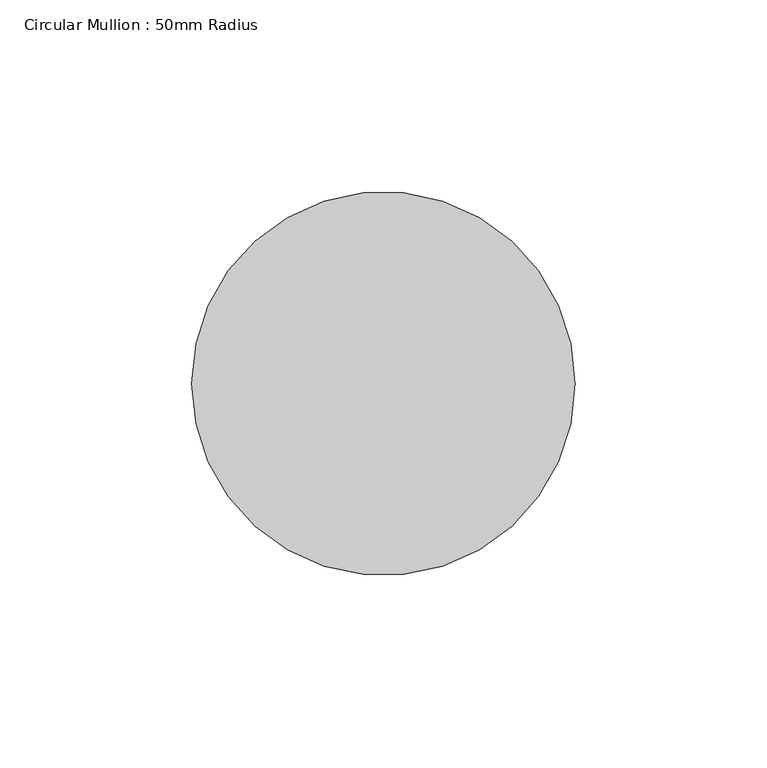
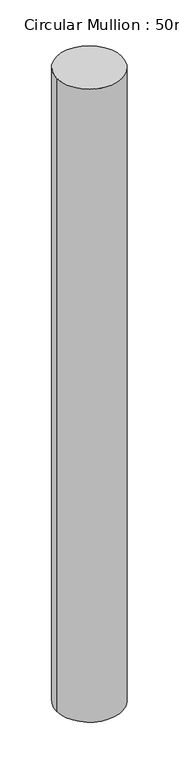
"""IFC4 building model written with IfcOpenShell, lengths in millimetres: member geometry, Circular Mullion : 50mm Radius."""

from ifc_helpers import new_model, si_unit, point, frame, origin, origin_2d, place, context, project, spatial, circle_curve, trimmed, segment, composite_curve, outline, extrude, source, transform, mapped, element, save


def circular_mullion_50mm_radius_72e26036(model_context):
    return source(origin(), model_context, "Body", "SweptSolid", [
        extrude(outline(composite_curve([segment(trimmed(circle_curve(origin_2d(), 50.0), [point((50.0, 0.0))], [point((-50.0, 0.0))], False, "CARTESIAN"), True, "CONTINUOUS"), segment(trimmed(circle_curve(origin_2d(), 50.0), [point((-50.0, 0.0))], [point((50.0, 0.0))], False, "CARTESIAN"), True, "CONTINUOUS")], self_intersect=False)), frame((0.0, 0.0, -1021.3712553), z_axis=(0.0, 0.0, 1.0), x_axis=(1.0, 0.0, 0.0)), (0.0, 0.0, 1.0), 1021.3712553),
    ])


if __name__ == "__main__":
    model = new_model("IFC4")
    model_context = context("Model", 3, world=origin())
    ifc_project = project(units=[si_unit("LENGTHUNIT", "METRE", prefix="MILLI")], contexts=[model_context])
    site = spatial("IfcSite", under=ifc_project)
    building = spatial("IfcBuilding", under=site)
    placement = place(None, origin())
    circular_mullion_50mm_radius_shape = circular_mullion_50mm_radius_72e26036(model_context)
    element("IfcMember", 1, ObjectType="Circular Mullion : 50mm Radius", at=placement, inside=building, context=model_context, shape_type="MappedRepresentation", body=[
        mapped(circular_mullion_50mm_radius_shape, transform((0.0, 0.0, 0.0), x_axis=(1.0, 0.0, 0.0), y_axis=(0.0, 1.0, 0.0), z_axis=(0.0, 0.0, 1.0))),
    ])
    save(model, "model.ifc")

# Revit data of these elements
# Type "Circular Mullion : 50mm Radius"
#   built-in parameter 1007350 = 0.164042 (stored number, unit not read)
# Element 1 (IfcMember, "Circular Mullion : 50mm Radius")
#   Materials on its faces: "Aluminium"
# Materials
#   "Aluminium": class "Metal", colour RGB 247 247 247, transparency 0, Description = "Aluminium 6061", Cost = 0
